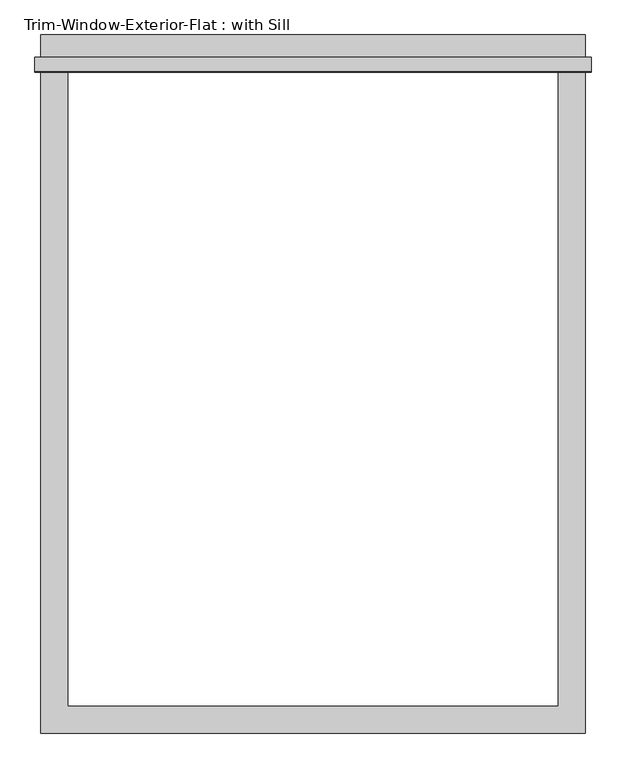
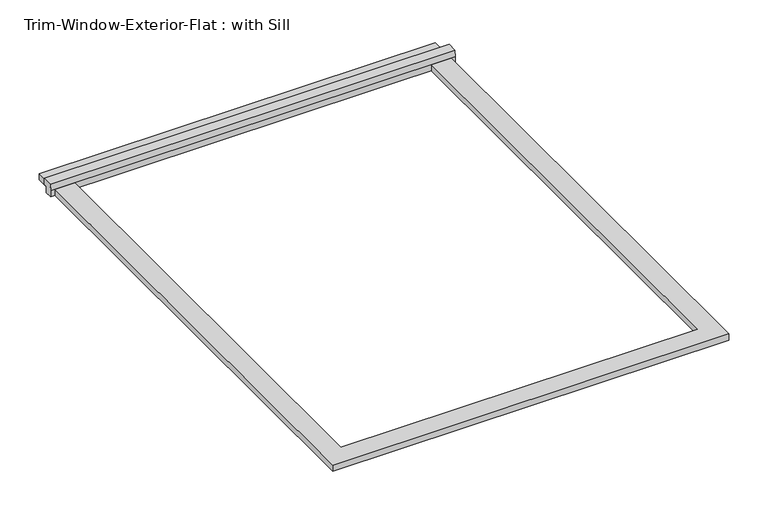
"""IFC4 building model written with IfcOpenShell, lengths in millimetres: proxy geometry, Trim-Window-Exterior-Flat : with Sill."""

from ifc_helpers import new_model, si_unit, frame, origin, origin_with_axes, place, context, project, spatial, polyline, outline, extrude, source, transform, mapped, element, save


def trim_window_exterior_flat_with_sill_076b70b5(model_context):
    return source(origin(), model_context, "Body", "SweptSolid", [
        extrude(outline(polyline([(577.85, 1368.3823709), (-577.85, 1368.3823709), (-577.85, 1425.5323709), (577.85, 1425.5323709), (577.85, 1368.3823709)])), origin_with_axes(), (0.0, 0.0, 1.0), 19.05),
        extrude(outline(polyline([(1377.95, 38.1), (1377.95, 19.05), (1368.3823709, 19.05), (1368.3823709, 0.0), (1346.2, 0.0), (1346.2, 19.05), (1348.6580645, 38.1), (1377.95, 38.1)])), frame((-590.55, 0.0, 0.0), z_axis=(1.0, 0.0, 0.0), x_axis=(0.0, 1.0, 0.0)), (0.0, 0.0, 1.0), 1181.1),
        extrude(outline(polyline([(-577.85, -57.15), (-577.85, 1346.2), (-520.7, 1346.2), (-520.7, 0.0), (520.7, 0.0), (520.7, 1346.2), (577.85, 1346.2), (577.85, -57.15), (-577.85, -57.15)])), origin_with_axes(), (0.0, 0.0, 1.0), 19.05),
    ])


if __name__ == "__main__":
    model = new_model("IFC4")
    model_context = context("Model", 3, world=origin())
    ifc_project = project(units=[si_unit("LENGTHUNIT", "METRE", prefix="MILLI")], contexts=[model_context])
    site = spatial("IfcSite", under=ifc_project)
    building = spatial("IfcBuilding", under=site)
    placement = place(None, origin())
    trim_window_exterior_flat_with_sill_shape = trim_window_exterior_flat_with_sill_076b70b5(model_context)
    element("IfcBuildingElementProxy", 1, Name="Trim-Window-Exterior-Flat : with Sill", ObjectType="Trim-Window-Exterior-Flat : with Sill", at=placement, inside=building, context=model_context, shape_type="MappedRepresentation", body=[
        mapped(trim_window_exterior_flat_with_sill_shape, transform((0.0, 0.0, 0.0), x_axis=(1.0, 0.0, 0.0), y_axis=(0.0, 1.0, 0.0), z_axis=(0.0, 0.0, 1.0))),
    ])
    save(model, "model.ifc")

# Revit data of these elements
# Project information
#   Project Issue Date = "Issue Date"
#   Project Status = "Project Status"
#   Client Name = "Owner"
#   Project Address = "Enter address here"
#   Project Name = "Project Name"
#   Project Number = "Project Number"
# Type "Trim-Window-Exterior-Flat : with Sill"
#   Trim Width = 0' - 2 1/4"
#   Trim Thickness_Picture Frame = 0' - 1 1/4"
#   Trim Thickness_with Sill = 0' - 0 3/4"
#   Sill Thickness = 0' - 1 1/4"
#   Opening Width [instance default] = 2' - 0"
#   Opening Height [instance default] = 3' - 0"
#   Default Elevation = 4' - 0"
#   Sill = yes
#   Picture Frame = no
#   Trim Material [instance default] = none
# Element 1 (IfcBuildingElementProxy, "Trim-Window-Exterior-Flat : with Sill")
#   Opening Width = 3' - 5"
#   Opening Height = 4' - 5"
#   Trim Material = Clad - White
#   Materials on its faces: "Clad - White"
# Materials
#   "Clad - White": class "Wood", colour RGB 216 216 204, transparency 0, Cost = 0
